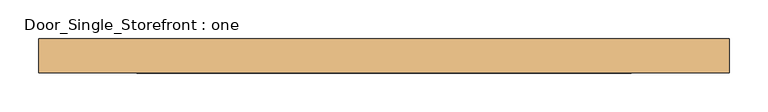
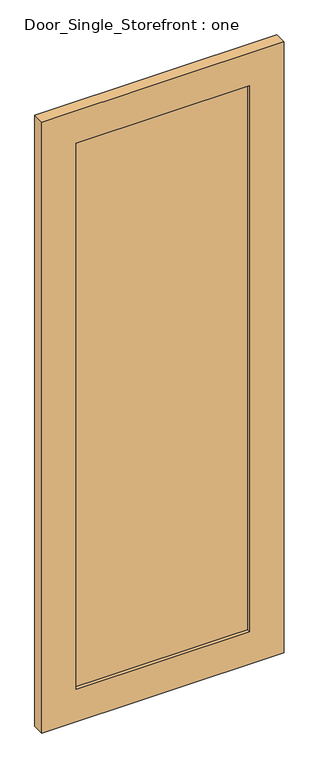
"""IFC4 building model written with IfcOpenShell, lengths in millimetres: door geometry, Door_Single_Storefront : one."""

from ifc_helpers import new_model, si_unit, frame, origin, place, context, project, spatial, polyline, outline, extrude, source, transform, mapped, element, save


def door_single_storefront_one_a28830f2(model_context):
    return source(origin(), model_context, "Body", "SweptSolid", [
        extrude(outline(polyline([(319.88125, 6.35), (319.88125, -12.7), (-319.88125, -12.7), (-319.88125, 6.35), (319.88125, 6.35)])), frame((0.0, 0.0, 127.0), z_axis=(0.0, 0.0, 1.0), x_axis=(1.0, 0.0, 0.0)), (0.0, 0.0, 1.0), 2127.25),
        extrude(outline(polyline([(2381.25, -446.88125), (0.0, -446.88125), (0.0, 446.88125), (2381.25, 446.88125), (2381.25, -446.88125)]), holes=[polyline([(127.0, 319.88125), (127.0, -319.88125), (2254.25, -319.88125), (2254.25, 319.88125), (127.0, 319.88125)])]), frame((0.0, -25.4, 0.0), z_axis=(0.0, 1.0, 0.0), x_axis=(0.0, 0.0, 1.0)), (0.0, 0.0, 1.0), 44.45),
    ])


if __name__ == "__main__":
    model = new_model("IFC4")
    model_context = context("Model", 3, world=origin())
    ifc_project = project(units=[si_unit("LENGTHUNIT", "METRE", prefix="MILLI")], contexts=[model_context])
    site = spatial("IfcSite", under=ifc_project)
    building = spatial("IfcBuilding", under=site)
    placement = place(None, origin())
    door_single_storefront_one_shape = door_single_storefront_one_a28830f2(model_context)
    element("IfcDoor", 1, ObjectType="Door_Single_Storefront : one", at=placement, inside=building, context=model_context, shape_type="MappedRepresentation", body=[
        mapped(door_single_storefront_one_shape, transform((0.0, 0.0, 0.0), x_axis=(1.0, 0.0, 0.0), y_axis=(0.0, 1.0, 0.0), z_axis=(0.0, 0.0, 1.0))),
    ])
    save(model, "model.ifc")

# Revit data of these elements
# Type "Door_Single_Storefront : one"
#   Type Mark = "27"
#   Analytic Construction = "<None>"
#   Stile_Width = 0' - 5"
#   Door_Thickness = 0' - 1 3/4"
#   Door_Offset = 0' - 1"
#   Glass_Material = SAFETY GLAZING
#   Frame_Material = INTERIOR GRADE ALUMINUM STOREFRONT W/ SAFETY GLAZING
#   Function = (empty or 0)
# Element 1 (IfcDoor, "Door_Single_Storefront : one")
#   Materials on its faces: "INTERIOR GRADE ALUMINUM STOREFRONT W/ SAFETY GLAZING", "SAFETY GLAZING"
# Materials
#   "SAFETY GLAZING": class "Glass", colour RGB 142 168 196, transparency 0.75, Description = "Soda Lime Glass", Cost = 0
#   "INTERIOR GRADE ALUMINUM STOREFRONT W/ SAFETY GLAZING": class "Metal", colour RGB 226 226 226, transparency 0, Description = "Aluminum 6061", Cost = 0
